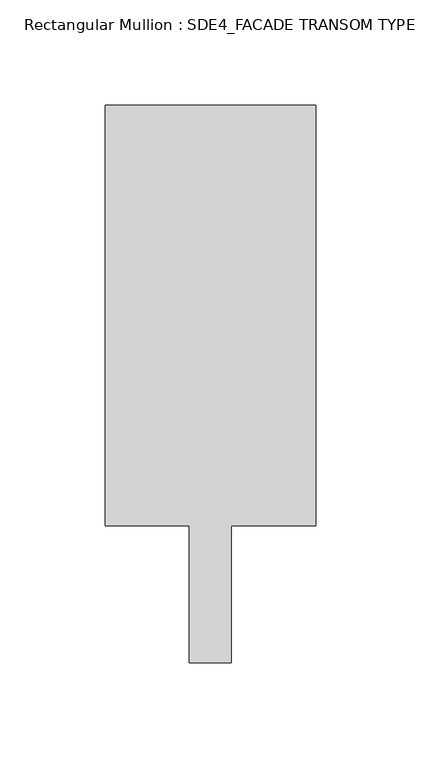
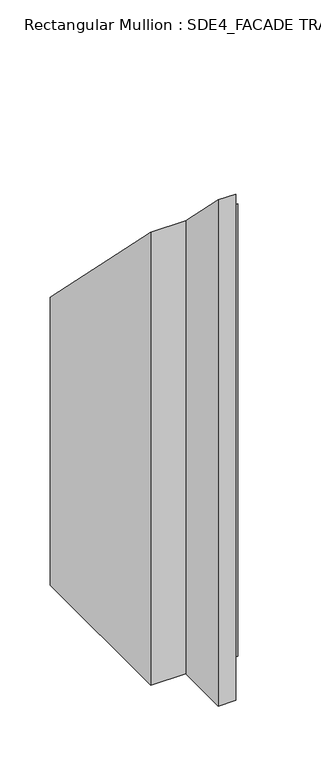
"""IFC4 building model written with IfcOpenShell, lengths in millimetres: member geometry, Rectangular Mullion : SDE4_FACADE TRANSOM TYPE 2."""

from ifc_helpers import new_model, si_unit, origin, place, context, project, spatial, faceted_brep, source, transform, mapped, element, save


def rectangular_mullion_sde4_facade_transom_type_2_0dbc9179(model_context):
    return source(origin(), model_context, "Body", "Brep", [
        faceted_brep([(50.0, 132.5, -482.4999945), (50.0, -67.5, -482.4999945), (10.0, -67.5, -482.4999945), (10.0, -132.5, -482.4999945), (-10.0, -132.5, -482.4999945), (-10.0, -67.5, -482.4999945), (-50.0, -67.5, -482.4999945), (-50.0, 132.5, -482.4999945), (-50.0, 132.5, -132.5), (50.0, 132.5, -132.5), (-50.0, -67.5, 67.5), (-10.0, -67.5, 67.5), (-10.0, -132.5, 132.5), (10.0, -132.5, 132.5), (10.0, -67.5, 67.5), (50.0, -67.5, 67.5)], [[[0, 1, 2, 3, 4, 5, 6, 7]], [[8, 9, 0, 7]], [[10, 8, 7, 6]], [[11, 10, 6, 5]], [[12, 11, 5, 4]], [[13, 12, 4, 3]], [[14, 13, 3, 2]], [[15, 14, 2, 1]], [[9, 15, 1, 0]], [[9, 8, 10, 11, 12, 13, 14, 15]]]),
    ])


if __name__ == "__main__":
    model = new_model("IFC4")
    model_context = context("Model", 3, world=origin())
    ifc_project = project(units=[si_unit("LENGTHUNIT", "METRE", prefix="MILLI")], contexts=[model_context])
    site = spatial("IfcSite", under=ifc_project)
    building = spatial("IfcBuilding", under=site)
    placement = place(None, origin())
    rectangular_mullion_sde4_facade_transom_type_2_shape = rectangular_mullion_sde4_facade_transom_type_2_0dbc9179(model_context)
    element("IfcMember", 1, ObjectType="Rectangular Mullion : SDE4_FACADE TRANSOM TYPE 2", at=placement, inside=building, context=model_context, shape_type="MappedRepresentation", body=[
        mapped(rectangular_mullion_sde4_facade_transom_type_2_shape, transform((0.0, 0.0, 0.0), x_axis=(1.0, 0.0, 0.0), y_axis=(0.0, 1.0, 0.0), z_axis=(0.0, 0.0, 1.0))),
    ])
    save(model, "model.ifc")

# Revit data of these elements
# Type "Rectangular Mullion : SDE4_FACADE TRANSOM TYPE 2"
#   built-in parameter 1007322 = 0.869423 (stored number, unit not read)
#   built-in parameter 1007321 = 0.164042 (stored number, unit not read)
#   built-in parameter 1007320 = 0.164042 (stored number, unit not read)
